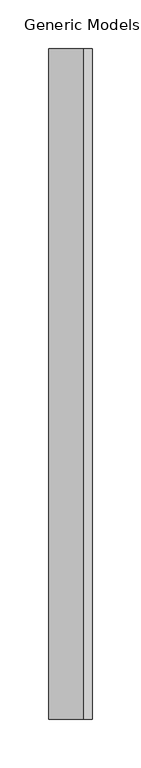
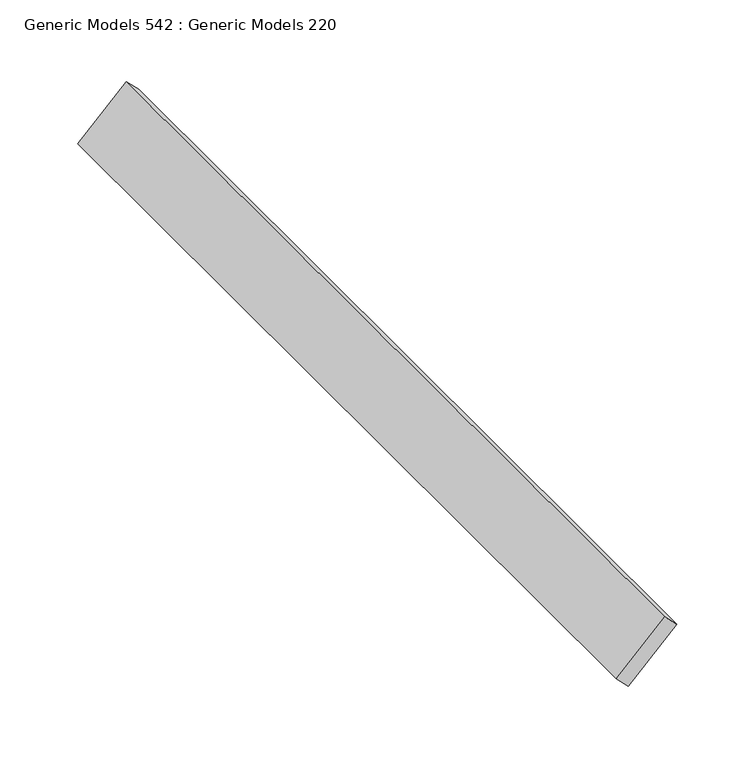
"""IFC4 building model written with IfcOpenShell, lengths in millimetres: proxy geometry, Generic Models 542 : Generic Models 220."""

from ifc_helpers import new_model, si_unit, frame, origin, place, context, project, spatial, polyline, outline, extrude, source, transform, mapped, element, save


def generic_models_542_generic_models_220_d128c7e6(model_context):
    return source(origin(), model_context, "Body", "SweptSolid", [
        extrude(outline(polyline([(0.0, -12.7000001), (0.0, 0.0), (690.8142348, 0.0), (690.8142348, -12.7000001), (0.0, -12.7000001)])), frame((7841.3059863, 4539.4872686, 124938.1399101), z_axis=(0.7071067811868034, 0.0, 0.7071067811862918), x_axis=(0.0, -1.0, 0.0)), (0.0, 0.0, 1.0), 50.8),
    ])


if __name__ == "__main__":
    model = new_model("IFC4")
    model_context = context("Model", 3, world=origin())
    ifc_project = project(units=[si_unit("LENGTHUNIT", "METRE", prefix="MILLI")], contexts=[model_context])
    site = spatial("IfcSite", under=ifc_project)
    building = spatial("IfcBuilding", under=site)
    placement = place(None, origin())
    generic_models_542_generic_models_220_shape = generic_models_542_generic_models_220_d128c7e6(model_context)
    element("IfcBuildingElementProxy", 1, Name="Generic Models 542 : Generic Models 220", ObjectType="Generic Models 542 : Generic Models 220", at=placement, inside=building, context=model_context, shape_type="MappedRepresentation", body=[
        mapped(generic_models_542_generic_models_220_shape, transform((0.0, 0.0, 0.0), x_axis=(1.0, 0.0, 0.0), y_axis=(0.0, 1.0, 0.0), z_axis=(0.0, 0.0, 1.0))),
    ])
    save(model, "model.ifc")

# Revit data of these elements
# Element 1 (IfcBuildingElementProxy, "Generic Models 542 : Generic Models 220")
#   Materials on its faces: "_WOOD TONE ALUMINUM EXTRUSION SLAT BY KNOTWOOD"
# Materials
#   "_WOOD TONE ALUMINUM EXTRUSION SLAT BY KNOTWOOD": class "Generic", colour RGB 177 130 114, transparency 0, Cost = 0
